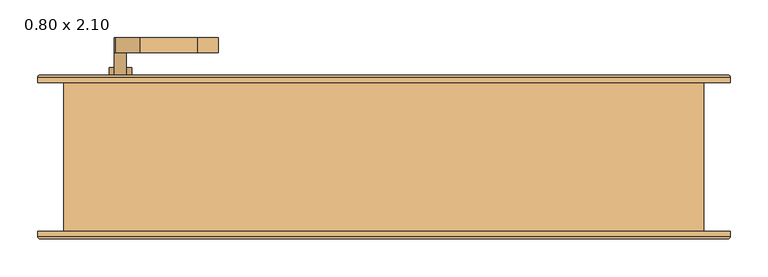
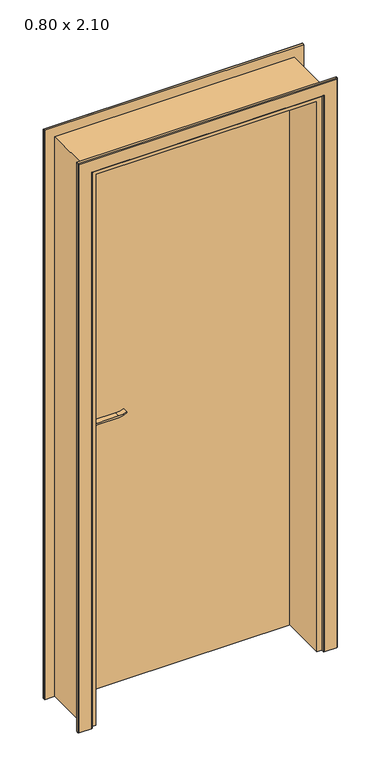
"""IFC4 building model written with IfcOpenShell, lengths in millimetres: door geometry, .CC_ND 300_PORTA SIMPLES DE ABRIR_COM EXTENSÃO : 0.80 x 2.10."""

from ifc_helpers import new_model, si_unit, point, frame, frame_2d, origin, origin_with_axes, place, context, project, spatial, polyline, circle_curve, ellipse_curve, trimmed, segment, composite_curve, outline, extrude, faceted_brep, source, transform, mapped, element, save
from ifc_brep_helpers import plane_surface, cylinder_surface, advanced_brep


def door_0_80_x_2_10_81f54b8d(model_context):
    return source(origin(), model_context, "Body", "SolidModel", [
        extrude(outline(composite_curve([segment(trimmed(circle_curve(frame_2d((964.5, -350.0)), 15.0), [point((964.5, -335.0))], [point((964.5, -365.0))], False, "CARTESIAN"), True, "CONTINUOUS"), segment(trimmed(circle_curve(frame_2d((964.5, -350.0)), 15.0), [point((964.5, -365.0))], [point((964.5, -335.0))], False, "CARTESIAN"), True, "CONTINUOUS")], self_intersect=False)), frame((0.0, 108.8, 0.0), z_axis=(0.0, 1.0, 0.0), x_axis=(0.0, 0.0, 1.0)), (0.0, 0.0, 1.0), 10.0),
        extrude(outline(composite_curve([segment(trimmed(circle_curve(frame_2d((964.5, -350.0)), 15.0), [point((964.5, -335.0))], [point((964.5, -365.0))], False, "CARTESIAN"), True, "CONTINUOUS"), segment(trimmed(circle_curve(frame_2d((964.5, -350.0)), 15.0), [point((964.5, -365.0))], [point((964.5, -335.0))], False, "CARTESIAN"), True, "CONTINUOUS")], self_intersect=False)), frame((0.0, 48.8, 0.0), z_axis=(0.0, 1.0, 0.0), x_axis=(0.0, 0.0, 1.0)), (0.0, 0.0, 1.0), 10.0),
        extrude(outline(composite_curve([segment(trimmed(circle_curve(frame_2d((1024.5, -350.0)), 8.0), [point((1029.1523287, -356.5081363))], [point((1024.5, -342.0))], False, "CARTESIAN"), True, "CONTINUOUS"), segment(trimmed(circle_curve(frame_2d((1019.3738613, -324.6138099)), 18.1261387), [point((1024.5, -342.0))], [point((1037.5, -324.6138099))], True, "CARTESIAN"), True, "CONTINUOUS"), segment(polyline([(1037.5, -324.6138099), (1037.5, -248.3564091)]), True, "CONTINUOUS"), segment(trimmed(circle_curve(frame_2d((1096.7709207, -251.9396612)), 59.3791355), [point((1037.5, -248.3564091))], [point((1046.7135558, -220.0))], False, "CARTESIAN"), True, "CONTINUOUS"), segment(polyline([(1046.7135558, -220.0), (1049.5, -220.0)]), True, "CONTINUOUS"), segment(trimmed(circle_curve(frame_2d((1127.7850638, -248.4227909)), 83.2850902), [point((1049.5, -220.0))], [point((1044.5, -248.3564091))], True, "CARTESIAN"), True, "CONTINUOUS"), segment(polyline([(1044.5, -248.3564091), (1044.5, -324.6325667)]), True, "CONTINUOUS"), segment(trimmed(circle_curve(frame_2d((1007.2555521, -326.3324871)), 37.2832219), [point((1044.5, -324.6325667))], [point((1029.1523287, -356.5081363))], False, "CARTESIAN"), True, "CONTINUOUS")], self_intersect=False)), frame((0.0, 138.8, 0.0), z_axis=(0.0, 1.0, 0.0), x_axis=(0.0, 0.0, 1.0)), (0.0, 0.0, 1.0), 20.0),
        extrude(outline(composite_curve([segment(trimmed(circle_curve(frame_2d((1019.3738682, -324.6138122)), 18.1261318), [point((1024.4999903, -342.0))], [point((1037.5, -324.6138122))], True, "CARTESIAN"), True, "CONTINUOUS"), segment(polyline([(1037.5, -324.6138122), (1037.5, -248.3564091)]), True, "CONTINUOUS"), segment(trimmed(circle_curve(frame_2d((1096.7709207, -251.9396612)), 59.3791355), [point((1037.5, -248.3564091))], [point((1046.7135558, -220.0))], False, "CARTESIAN"), True, "CONTINUOUS"), segment(polyline([(1046.7135558, -220.0), (1049.5, -220.0)]), True, "CONTINUOUS"), segment(trimmed(circle_curve(frame_2d((1127.7850638, -248.4227909)), 83.2850902), [point((1049.5, -220.0))], [point((1044.5, -248.3564091))], True, "CARTESIAN"), True, "CONTINUOUS"), segment(polyline([(1044.5, -248.3564091), (1044.5, -324.6325667)]), True, "CONTINUOUS"), segment(trimmed(circle_curve(frame_2d((1007.2555521, -326.3324871)), 37.2832219), [point((1044.5, -324.6325667))], [point((1029.1523287, -356.5081363))], False, "CARTESIAN"), True, "CONTINUOUS"), segment(trimmed(circle_curve(frame_2d((1024.5, -350.0)), 8.0), [point((1029.1523287, -356.5081363))], [point((1024.4999903, -342.0))], False, "CARTESIAN"), True, "CONTINUOUS")], self_intersect=False)), frame((0.0, 8.8, 0.0), z_axis=(0.0, 1.0, 0.0), x_axis=(0.0, 0.0, 1.0)), (0.0, 0.0, 1.0), 20.0),
        extrude(outline(composite_curve([segment(trimmed(circle_curve(frame_2d((1024.5, -350.0)), 8.0), [point((1024.5, -342.0))], [point((1024.5, -358.0))], False, "CARTESIAN"), True, "CONTINUOUS"), segment(trimmed(circle_curve(frame_2d((1024.5, -350.0)), 8.0), [point((1024.5, -358.0))], [point((1024.5, -342.0))], False, "CARTESIAN"), True, "CONTINUOUS")], self_intersect=False)), frame((0.0, 108.8, 0.0), z_axis=(0.0, 1.0, 0.0), x_axis=(0.0, 0.0, 1.0)), (0.0, 0.0, 1.0), 30.0),
        extrude(outline(composite_curve([segment(trimmed(circle_curve(frame_2d((1024.5, -350.0)), 8.0), [point((1024.5, -342.0))], [point((1024.5, -358.0))], False, "CARTESIAN"), True, "CONTINUOUS"), segment(trimmed(circle_curve(frame_2d((1024.5, -350.0)), 8.0), [point((1024.5, -358.0))], [point((1024.5, -342.0))], False, "CARTESIAN"), True, "CONTINUOUS")], self_intersect=False)), frame((0.0, 28.8, 0.0), z_axis=(0.0, 1.0, 0.0), x_axis=(0.0, 0.0, 1.0)), (0.0, 0.0, 1.0), 30.0),
        extrude(outline(composite_curve([segment(trimmed(circle_curve(frame_2d((954.5, -350.0)), 25.0), [point((954.5, -375.0))], [point((954.5, -325.0))], False, "CARTESIAN"), True, "CONTINUOUS"), segment(polyline([(954.5, -325.0), (1024.5, -325.0)]), True, "CONTINUOUS"), segment(trimmed(circle_curve(frame_2d((1024.5, -350.0)), 25.0), [point((1024.5, -325.0))], [point((1024.5, -375.0))], False, "CARTESIAN"), True, "CONTINUOUS"), segment(polyline([(1024.5, -375.0), (954.5, -375.0)]), True, "CONTINUOUS")], self_intersect=False)), frame((0.0, 98.8, 0.0), z_axis=(0.0, 1.0, 0.0), x_axis=(0.0, 0.0, 1.0)), (0.0, 0.0, 1.0), 10.0),
        extrude(outline(composite_curve([segment(trimmed(circle_curve(frame_2d((954.5, -350.0)), 25.0), [point((954.5, -375.0))], [point((954.5, -325.0))], False, "CARTESIAN"), True, "CONTINUOUS"), segment(polyline([(954.5, -325.0), (1024.5, -325.0)]), True, "CONTINUOUS"), segment(trimmed(circle_curve(frame_2d((1024.5, -350.0)), 25.0), [point((1024.5, -325.0))], [point((1024.5, -375.0))], False, "CARTESIAN"), True, "CONTINUOUS"), segment(polyline([(1024.5, -375.0), (954.5, -375.0)]), True, "CONTINUOUS")], self_intersect=False)), frame((0.0, 58.8, 0.0), z_axis=(0.0, 1.0, 0.0), x_axis=(0.0, 0.0, 1.0)), (0.0, 0.0, 1.0), 10.0),
        faceted_brep([(392.0, -98.8, 0.0), (392.0, 68.8, 0.0), (400.0, 68.8, 0.0), (400.0, 98.8, 0.0), (425.0, 98.8, 0.0), (425.0, -98.8, 0.0), (425.0, -98.8, 2100.0), (-425.0, -98.8, 2100.0), (-425.0, -98.8, 0.0), (-392.0, -98.8, 0.0), (-392.0, -98.8, 2067.0), (392.0, -98.8, 2067.0), (425.0, 98.8, 2100.0), (400.0, 98.8, 2075.0), (-400.0, 98.8, 2075.0), (-400.0, 98.8, 0.0), (-425.0, 98.8, 0.0), (-425.0, 98.8, 2100.0), (400.0, 68.8, 2075.0), (392.0, 68.8, 2067.0), (-392.0, 68.8, 2067.0), (-392.0, 68.8, 0.0), (-400.0, 68.8, 0.0), (-400.0, 68.8, 2075.0)], [[[0, 1, 2, 3, 4, 5]], [[5, 6, 7, 8, 9, 10, 11, 0]], [[4, 12, 6, 5]], [[3, 13, 14, 15, 16, 17, 12, 4]], [[2, 18, 13, 3]], [[1, 19, 20, 21, 22, 23, 18, 2]], [[0, 11, 19, 1]], [[10, 9, 21, 20]], [[9, 8, 16, 15, 22, 21]], [[17, 16, 8, 7]], [[23, 22, 15, 14]], [[12, 17, 7, 6]], [[18, 23, 14, 13]], [[11, 10, 20, 19]]]),
        extrude(outline(polyline([(-400.0, 68.8), (-400.0, 98.8), (400.0, 98.8), (400.0, 68.8), (-400.0, 68.8)])), origin_with_axes(), (0.0, 0.0, 1.0), 2075.0),
        advanced_brep(
        [(-460.0, 98.8, 0.0), (-460.0, 105.8, 0.0), (-457.0, 108.8, 0.0), (-413.0, 108.8, 0.0), (-410.0, 105.8, 0.0), (-410.0, 98.8, 0.0), (-410.0, 98.8, 2085.0), (410.0, 98.8, 2085.0), (410.0, 98.8, 0.0), (460.0, 98.8, 0.0), (460.0, 98.8, 2135.0), (-460.0, 98.8, 2135.0), (-410.0, 105.8, 2085.0), (-413.0, 108.8, 2088.0), (-457.0, 108.8, 2132.0), (457.0, 108.8, 2132.0), (457.0, 108.8, 0.0), (413.0, 108.8, 0.0), (413.0, 108.8, 2088.0), (-460.0, 105.8, 2135.0), (460.0, 105.8, 0.0), (460.0, 105.8, 2135.0), (410.0, 105.8, 0.0), (410.0, 105.8, 2085.0)],
        [
            (0, 1),
            (1, 2, circle_curve(frame((-457.0, 105.8, 0.0), z_axis=(0.0, 0.0, -1.0), x_axis=(1.0, 0.0, 0.0)), 3.0)),
            (2, 3),
            (3, 4, circle_curve(frame((-413.0, 105.8, 0.0), z_axis=(0.0, 0.0, -1.0), x_axis=(1.0, 0.0, 0.0)), 3.0)),
            (4, 5),
            (5, 0),
            (5, 6),
            (6, 7),
            (7, 8),
            (8, 9),
            (9, 10),
            (10, 11),
            (11, 0),
            (4, 12),
            (12, 6),
            (3, 13),
            (13, 12, ellipse_curve(frame((-413.0, 105.8, 2088.0), z_axis=(-0.7071067811865475, 0.0, -0.7071067811865475), x_axis=(0.7071067811865474, 0.0, -0.7071067811865476)), 4.2426407, 3.0)),
            (2, 14),
            (14, 15),
            (15, 16),
            (16, 17),
            (17, 18),
            (18, 13),
            (1, 19),
            (19, 14, ellipse_curve(frame((-457.0, 105.8, 2132.0), z_axis=(-0.7071067811865475, 0.0, -0.7071067811865475), x_axis=(0.7071067811865474, 0.0, -0.7071067811865476)), 4.2426407, 3.0)),
            (11, 19),
            (9, 20),
            (20, 21),
            (21, 10),
            (8, 22),
            (22, 17, circle_curve(frame((413.0, 105.8, 0.0), z_axis=(0.0, 0.0, -1.0), x_axis=(-1.0, 0.0, 0.0)), 3.0)),
            (16, 20, circle_curve(frame((457.0, 105.8, 0.0), z_axis=(0.0, 0.0, -1.0), x_axis=(-1.0, 0.0, 0.0)), 3.0)),
            (23, 22),
            (7, 23),
            (23, 18, ellipse_curve(frame((413.0, 105.8, 2088.0), z_axis=(0.7071067811865475, 0.0, -0.7071067811865475), x_axis=(0.7071067811865474, 0.0, 0.7071067811865476)), 4.2426407, 3.0)),
            (15, 21, ellipse_curve(frame((457.0, 105.8, 2132.0), z_axis=(0.7071067811865475, 0.0, -0.7071067811865475), x_axis=(0.7071067811865474, 0.0, 0.7071067811865476)), 4.2426407, 3.0)),
            (12, 23),
            (21, 19),
        ],
        [
            plane_surface(frame((-410.0, 98.8, 0.0), z_axis=(0.0, 0.0, -1.0), x_axis=(0.0, -1.0, 0.0))),
            plane_surface(frame((-460.0, 98.8, 0.0), z_axis=(0.0, -1.0, 0.0), x_axis=(0.0, 0.0, 1.0))),
            plane_surface(frame((-410.0, 98.8, 0.0), z_axis=(1.0, 0.0, 0.0), x_axis=(0.0, 0.0, 1.0))),
            cylinder_surface(frame((-413.0, 105.8, 0.0), z_axis=(0.0, 0.0, -1.0), x_axis=(1.0, 0.0, 0.0)), 3.0),
            plane_surface(frame((-413.0, 108.8, 0.0), z_axis=(0.0, 1.0, 0.0), x_axis=(0.0, 0.0, 1.0))),
            cylinder_surface(frame((-457.0, 105.8, 0.0), z_axis=(0.0, 0.0, -1.0), x_axis=(1.0, 0.0, 0.0)), 3.0),
            plane_surface(frame((-460.0, 105.8, 0.0), z_axis=(-1.0, 0.0, 0.0), x_axis=(0.0, 0.0, 1.0))),
            plane_surface(frame((460.0, 105.8, 2135.0), z_axis=(1.0, 0.0, 0.0), x_axis=(0.0, 0.0, -1.0))),
            plane_surface(frame((410.0, 98.8, 0.0), z_axis=(0.0, 0.0, -1.0), x_axis=(0.0, -1.0, 0.0))),
            plane_surface(frame((410.0, 98.8, 2085.0), z_axis=(-1.0, 0.0, 0.0), x_axis=(0.0, 0.0, -1.0))),
            cylinder_surface(frame((413.0, 105.8, 2085.0), z_axis=(0.0, 0.0, 1.0), x_axis=(-1.0, 0.0, 0.0)), 3.0),
            cylinder_surface(frame((457.0, 105.8, 2085.0), z_axis=(0.0, 0.0, 1.0), x_axis=(-1.0, 0.0, 0.0)), 3.0),
            plane_surface(frame((-410.0, 98.8, 2085.0), z_axis=(0.0, 0.0, -1.0), x_axis=(1.0, 0.0, 0.0))),
            plane_surface(frame((-460.0, 105.8, 2135.0), z_axis=(0.0, 0.0, 1.0), x_axis=(1.0, 0.0, 0.0))),
            cylinder_surface(frame((-410.0, 105.8, 2088.0), z_axis=(-1.0, 0.0, 0.0), x_axis=(0.0, 0.0, -1.0)), 3.0),
            cylinder_surface(frame((-410.0, 105.8, 2132.0), z_axis=(-1.0, 0.0, 0.0), x_axis=(0.0, 0.0, -1.0)), 3.0),
        ],
        [
            (0, [[1, 2, 3, 4, 5, 6]]),
            (1, [[7, 8, 9, 10, 11, 12, 13, -6]]),
            (2, [[14, 15, -7, -5]]),
            (3, [[16, 17, -14, -4]]),
            (4, [[18, 19, 20, 21, 22, 23, -16, -3]]),
            (5, [[24, 25, -18, -2]]),
            (6, [[-13, 26, -24, -1]]),
            (7, [[-11, 27, 28, 29]]),
            (8, [[-10, 30, 31, -21, 32, -27]]),
            (9, [[33, -30, -9, 34]]),
            (10, [[-22, -31, -33, 35]]),
            (11, [[-28, -32, -20, 36]]),
            (12, [[37, -34, -8, -15]]),
            (13, [[-12, -29, 38, -26]]),
            (14, [[-23, -35, -37, -17]]),
            (15, [[-38, -36, -19, -25]]),
        ],
    ),
        advanced_brep(
        [(460.0, -98.8, 0.0), (460.0, -105.8342217, 0.0), (457.0342217, -108.8, 0.0), (412.9842717, -108.8, 0.0), (410.0, -105.8157283, 0.0), (410.0, -98.8, 0.0), (410.0, -98.8, 2085.0), (-410.0, -98.8, 2085.0), (-410.0, -98.8, 0.0), (-460.0, -98.8, 0.0), (-460.0, -98.8, 2135.0), (460.0, -98.8, 2135.0), (410.0, -105.8157283, 2085.0), (412.9842717, -108.8, 2087.9842717), (457.0342217, -108.8, 2132.0342217), (-457.0342217, -108.8, 2132.0342217), (-457.0342217, -108.8, 0.0), (-412.9842717, -108.8, 0.0), (-412.9842717, -108.8, 2087.9842717), (460.0, -105.8342217, 2135.0), (-460.0, -105.8342217, 0.0), (-460.0, -105.8342217, 2135.0), (-410.0, -105.8157283, 0.0), (-410.0, -105.8157283, 2085.0)],
        [
            (0, 1),
            (1, 2, circle_curve(frame((457.0342217, -105.8342217, 0.0), z_axis=(0.0, 0.0, -1.0), x_axis=(1.0, 0.0, 0.0)), 2.9657783)),
            (2, 3),
            (3, 4, circle_curve(frame((412.9842717, -105.8157283, 0.0), z_axis=(0.0, 0.0, -1.0), x_axis=(1.0, 0.0, 0.0)), 2.9842717)),
            (4, 5),
            (5, 0),
            (5, 6),
            (6, 7),
            (7, 8),
            (8, 9),
            (9, 10),
            (10, 11),
            (11, 0),
            (4, 12),
            (12, 6),
            (3, 13),
            (13, 12, ellipse_curve(frame((412.9842717, -105.8157283, 2087.9842717), z_axis=(0.7071067811865475, 0.0, -0.7071067811865475), x_axis=(-0.7071067811865474, 0.0, -0.7071067811865476)), 4.2203975, 2.9842717)),
            (2, 14),
            (14, 15),
            (15, 16),
            (16, 17),
            (17, 18),
            (18, 13),
            (1, 19),
            (19, 14, ellipse_curve(frame((457.0342217, -105.8342217, 2132.0342217), z_axis=(0.7071067811865475, 0.0, -0.7071067811865475), x_axis=(-0.7071067811865474, 0.0, -0.7071067811865476)), 4.1942438, 2.9657783)),
            (11, 19),
            (9, 20),
            (20, 21),
            (21, 10),
            (8, 22),
            (22, 17, circle_curve(frame((-412.9842717, -105.8157283, 0.0), z_axis=(0.0, 0.0, -1.0), x_axis=(-1.0, 0.0, 0.0)), 2.9842717)),
            (16, 20, circle_curve(frame((-457.0342217, -105.8342217, 0.0), z_axis=(0.0, 0.0, -1.0), x_axis=(-1.0, 0.0, 0.0)), 2.9657783)),
            (23, 22),
            (7, 23),
            (23, 18, ellipse_curve(frame((-412.9842717, -105.8157283, 2087.9842717), z_axis=(-0.7071067811865475, 0.0, -0.7071067811865475), x_axis=(-0.7071067811865474, 0.0, 0.7071067811865476)), 4.2203975, 2.9842717)),
            (15, 21, ellipse_curve(frame((-457.0342217, -105.8342217, 2132.0342217), z_axis=(-0.7071067811865475, 0.0, -0.7071067811865475), x_axis=(-0.7071067811865474, 0.0, 0.7071067811865476)), 4.1942438, 2.9657783)),
            (12, 23),
            (21, 19),
        ],
        [
            plane_surface(frame((410.0, -98.8, 0.0), z_axis=(0.0, 0.0, -1.0), x_axis=(0.0, -1.0, 0.0))),
            plane_surface(frame((460.0, -98.8, 0.0), z_axis=(0.0, 1.0, 0.0), x_axis=(0.0, 0.0, 1.0))),
            plane_surface(frame((410.0, -98.8, 0.0), z_axis=(-1.0, 0.0, 0.0), x_axis=(0.0, 0.0, 1.0))),
            cylinder_surface(frame((412.9842717, -105.8157283, 0.0), z_axis=(0.0, 0.0, -1.0), x_axis=(1.0, 0.0, 0.0)), 2.9842717),
            plane_surface(frame((412.9842717, -108.8, 0.0), z_axis=(0.0, -1.0, 0.0), x_axis=(0.0, 0.0, 1.0))),
            cylinder_surface(frame((457.0342217, -105.8342217, 0.0), z_axis=(0.0, 0.0, -1.0), x_axis=(1.0, 0.0, 0.0)), 2.9657783),
            plane_surface(frame((460.0, -105.8342217, 0.0), z_axis=(1.0, 0.0, 0.0), x_axis=(0.0, 0.0, 1.0))),
            plane_surface(frame((-460.0, -105.8342217, 2135.0), z_axis=(-1.0, 0.0, 0.0), x_axis=(0.0, 0.0, -1.0))),
            plane_surface(frame((-410.0, -98.8, 0.0), z_axis=(0.0, 0.0, -1.0), x_axis=(0.0, -1.0, 0.0))),
            plane_surface(frame((-410.0, -98.8, 2085.0), z_axis=(1.0, 0.0, 0.0), x_axis=(0.0, 0.0, -1.0))),
            cylinder_surface(frame((-412.9842717, -105.8157283, 2085.0), z_axis=(0.0, 0.0, 1.0), x_axis=(-1.0, 0.0, 0.0)), 2.9842717),
            cylinder_surface(frame((-457.0342217, -105.8342217, 2085.0), z_axis=(0.0, 0.0, 1.0), x_axis=(-1.0, 0.0, 0.0)), 2.9657783),
            plane_surface(frame((410.0, -98.8, 2085.0), z_axis=(0.0, 0.0, -1.0), x_axis=(-1.0, 0.0, 0.0))),
            plane_surface(frame((460.0, -105.8342217, 2135.0), z_axis=(0.0, 0.0, 1.0), x_axis=(-1.0, 0.0, 0.0))),
            cylinder_surface(frame((410.0, -105.8157283, 2087.9842717), z_axis=(1.0, 0.0, 0.0), x_axis=(0.0, 0.0, 1.0)), 2.9842717),
            cylinder_surface(frame((410.0, -105.8342217, 2132.0342217), z_axis=(1.0, 0.0, 0.0), x_axis=(0.0, 0.0, 1.0)), 2.9657783),
        ],
        [
            (0, [[1, 2, 3, 4, 5, 6]]),
            (1, [[7, 8, 9, 10, 11, 12, 13, -6]]),
            (2, [[14, 15, -7, -5]]),
            (3, [[16, 17, -14, -4]]),
            (4, [[18, 19, 20, 21, 22, 23, -16, -3]]),
            (5, [[24, 25, -18, -2]]),
            (6, [[-13, 26, -24, -1]]),
            (7, [[-11, 27, 28, 29]]),
            (8, [[-10, 30, 31, -21, 32, -27]]),
            (9, [[33, -30, -9, 34]]),
            (10, [[-22, -31, -33, 35]]),
            (11, [[-28, -32, -20, 36]]),
            (12, [[37, -34, -8, -15]]),
            (13, [[-12, -29, 38, -26]]),
            (14, [[-23, -35, -37, -17]]),
            (15, [[-38, -36, -19, -25]]),
        ],
    ),
    ])


if __name__ == "__main__":
    model = new_model("IFC4")
    model_context = context("Model", 3, world=origin())
    ifc_project = project(units=[si_unit("LENGTHUNIT", "METRE", prefix="MILLI")], contexts=[model_context])
    site = spatial("IfcSite", under=ifc_project)
    building = spatial("IfcBuilding", under=site)
    placement = place(None, origin())
    door_0_80_x_2_10_shape = door_0_80_x_2_10_81f54b8d(model_context)
    element("IfcDoor", 1, ObjectType=".CC_ND 300_PORTA SIMPLES DE ABRIR_COM EXTENSÃO : 0.80 x 2.10", at=placement, inside=building, context=model_context, shape_type="MappedRepresentation", body=[
        mapped(door_0_80_x_2_10_shape, transform((0.0, 0.0, 0.0), x_axis=(1.0, 0.0, 0.0), y_axis=(0.0, 1.0, 0.0), z_axis=(0.0, 0.0, 1.0))),
    ])
    save(model, "model.ifc")

# Revit data of these elements
# Type ".CC_ND 300_PORTA SIMPLES DE ABRIR_COM EXTENSÃO : 0.80 x 2.10"
#   Type Mark = "153"
#   Analytic Construction = "<None>"
#   Rough Width = 0.85 m
#   Espessura moldura externa = 0.01 m
#   Espessura moldura interna = 0.01 m
#   Largura moldura = 0.05 m
#   Extensão acabamento exterior [instance default] = 0.00 m
#   Extensão acabamento interior [instance default] = 0.00 m
#   Espessura batente = 0.025 m
#   Thickness = 0.03 m
#   Altura batente = 2.085 m
#   Aux Arco [instance default] = 0.80 m
#   Rough Height = 2.125 m
#   Height = 2.10 m
#   Width = 0.80 m
#   Moldura interna [instance default] = yes
#   Moldura externa [instance default] = yes
#   Porta = .MADEIRA COM PINTURA ESMALTE BRANCO ACETINADO
#   Moldura = .MADEIRA COM PINTURA ESMALTE BRANCO ACETINADO
#   Maçaneta = .ALUMÍNIO
#   Batente = .MADEIRA COM PINTURA ESMALTE BRANCO ACETINADO
#   Function = (empty or 0)
#   Wall Closure = (empty or 0)
# Element 1 (IfcDoor, ".CC_ND 300_PORTA SIMPLES DE ABRIR_COM EXTENSÃO : 0.80 x 2.10")
#   Materials on its faces: ".MADEIRA COM PINTURA ESMALTE BRANCO ACETINADO", ".ALUMÍNIO"
# Materials
#   ".MADEIRA COM PINTURA ESMALTE BRANCO ACETINADO": class ".CC_MADEIRAS", colour RGB 240 240 240, transparency 0, Description = "Madeira com pintura esmalte branco acetinado.", Cost = 0
#   ".ALUMÍNIO": class "CC_METAIS", colour RGB 244 244 244, transparency 0, Description = "Material alumínio", Cost = 0
